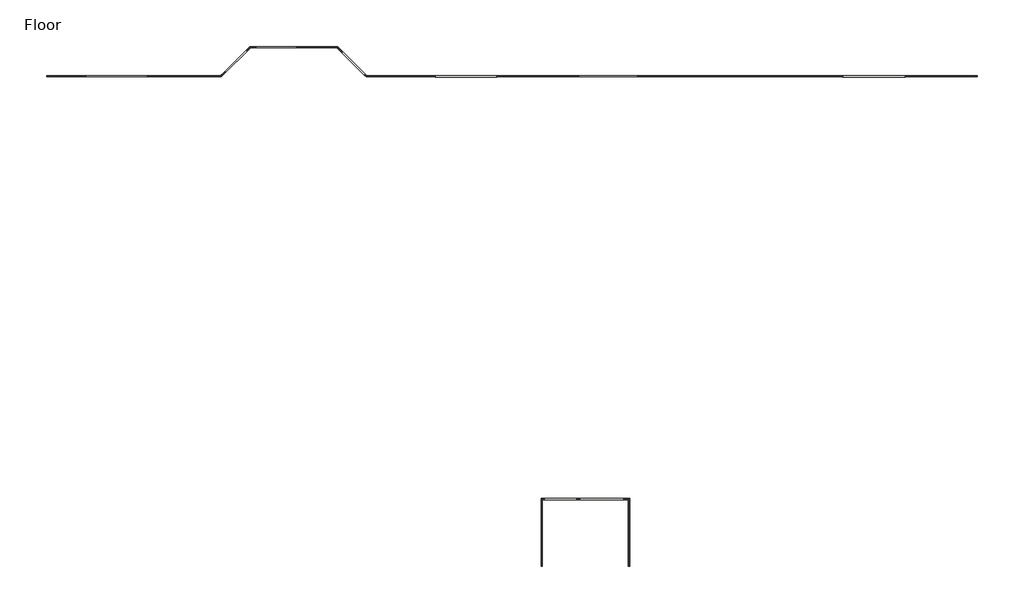
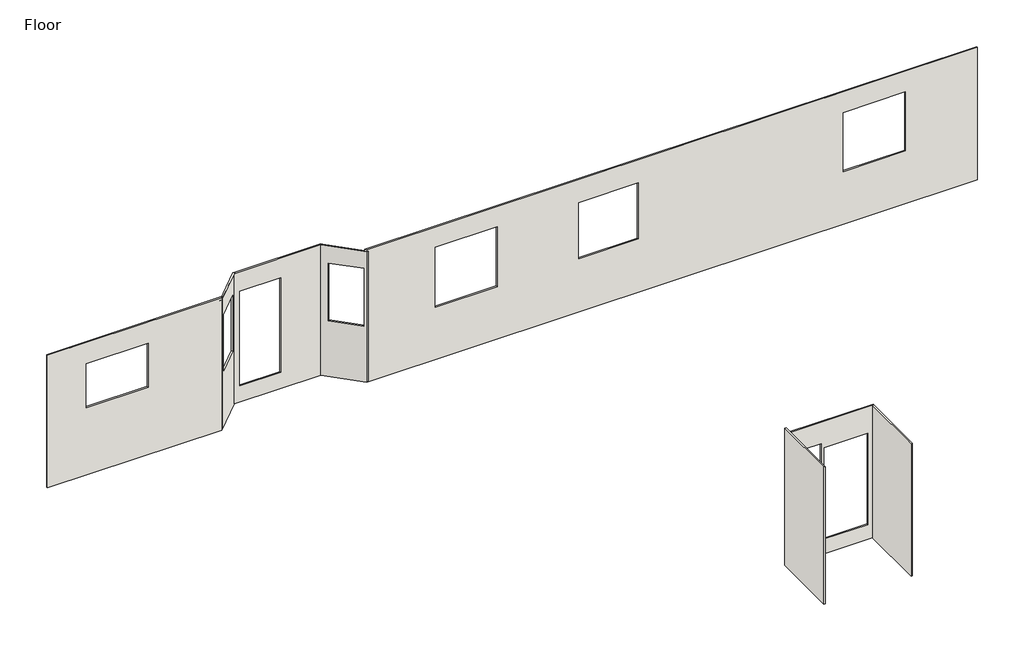
# One storey: 8 walls.
"""IFC4 building model written with IfcOpenShell, lengths in millimetres."""

import ifcopenshell
import ifcopenshell.guid

model = None  # the IFC model being written
_history = None  # IfcOwnerHistory: only IFC2X3 demands one
_inside = {}  # id of a spatial element -> (the spatial element, [elements in it])
_under = {}  # id of a project, library or spatial element -> (it, [spatial elements below it])
_declared = {}  # id of a project -> (the project, [libraries it declares])
_typed = {}  # id of a type object -> (the type object, [elements of that type])
_made_of = {}  # id of a material, layer set ... -> (it, [elements and type objects made of it])


def new_model(schema):
    """Start an empty IFC model of exactly this schema.

    Asked for "IFC4X3", IfcOpenShell would pick the latest addendum, in which some entities
    have other attributes; the version numbers below select the first issue.
    IFC2X3 requires an IfcOwnerHistory on every rooted entity: one is made here for all.
    """
    global model, _history
    if schema == "IFC4X3":
        model = ifcopenshell.file(schema_version=(4, 3, 0, 0))
    else:
        model = ifcopenshell.file(schema=schema)
    _inside.clear()
    _under.clear()
    _declared.clear()
    _typed.clear()
    _made_of.clear()
    _history = None
    if model.schema == "IFC2X3":
        org = make("IfcOrganization", Name="unknown")
        user = make(
            "IfcPersonAndOrganization",
            ThePerson=make("IfcPerson", FamilyName="unknown"),
            TheOrganization=org,
        )
        app = make(
            "IfcApplication",
            ApplicationDeveloper=org,
            Version="unknown",
            ApplicationFullName="unknown",
            ApplicationIdentifier="unknown",
        )
        _history = make(
            "IfcOwnerHistory",
            OwningUser=user,
            OwningApplication=app,
            ChangeAction="ADDED",
            CreationDate=0,
        )
    return model


def make(cls, **values):
    """One entity of the class cls with the attributes given. An attribute that is None is left unset."""
    return model.create_entity(
        cls, **{name: value for name, value in values.items() if value is not None}
    )


def rooted(cls, **values):
    """An entity with a GlobalId (a new one), such as an element, a storey or a relation."""
    return make(cls, GlobalId=ifcopenshell.guid.new(), OwnerHistory=_history, **values)


def si_unit(unit_type, name, prefix=None):
    """IfcSIUnit, for example si_unit("LENGTHUNIT", "METRE", prefix="MILLI")."""
    return make("IfcSIUnit", UnitType=unit_type, Prefix=prefix, Name=name)


def assignment(units):
    """IfcUnitAssignment: the units of a project."""
    return None if units is None else make("IfcUnitAssignment", Units=units)


def point(xyz):
    """IfcCartesianPoint."""
    return None if xyz is None else make("IfcCartesianPoint", Coordinates=xyz)


def direction(xyz):
    """IfcDirection."""
    return None if xyz is None else make("IfcDirection", DirectionRatios=xyz)


def frame(location, z_axis=None, x_axis=None):
    """IfcAxis2Placement3D, a coordinate frame: its origin and axes. An axis left out is left unset."""
    return make(
        "IfcAxis2Placement3D",
        Location=point(location),
        Axis=direction(z_axis),
        RefDirection=direction(x_axis),
    )


def origin():
    """The frame at (0, 0, 0) with its axes left unset."""
    return frame((0.0, 0.0, 0.0))


def place(relative_to, where):
    """IfcLocalPlacement: puts the frame where relative to a parent placement (None: the world)."""
    return make(
        "IfcLocalPlacement", PlacementRelTo=relative_to, RelativePlacement=where
    )


def context(
    kind, dimensions, precision=None, world=None, true_north=None, identifier=None
):
    """IfcGeometricRepresentationContext, for example the 3D "Model" context."""
    return make(
        "IfcGeometricRepresentationContext",
        ContextIdentifier=identifier,
        ContextType=kind,
        CoordinateSpaceDimension=dimensions,
        Precision=precision,
        WorldCoordinateSystem=world,
        TrueNorth=true_north,
    )


def project(units=None, contexts=None):
    """IfcProject with its units and contexts."""
    return rooted(
        "IfcProject",
        Name="project",
        RepresentationContexts=contexts,
        UnitsInContext=assignment(units),
    )


def spatial(cls, under=None, at=None, **own):
    """A site, building, storey or space (cls), placed at a placement, below another one or the project."""
    s = rooted(cls, ObjectPlacement=at, **own)
    if under is not None:
        _under.setdefault(under.id(), (under, []))[1].append(s)
    return s


def faces_of(points, faces, orient=None, outer=None):
    """IfcFace entities. A face is a list of loops; a loop is a list of indices into points, from 0.

    orient and outer hold one flag for each loop. By default every Orientation is true, the
    first loop of a face is its IfcFaceOuterBound and the others are IfcFaceBound.
    """
    made = []
    for i, loops in enumerate(faces):
        bounds = []
        for j, loop in enumerate(loops):
            is_outer = j == 0 if outer is None else outer[i][j]
            bounds.append(
                make(
                    "IfcFaceOuterBound" if is_outer else "IfcFaceBound",
                    Bound=make("IfcPolyLoop", Polygon=[points[k] for k in loop]),
                    Orientation=True if orient is None else orient[i][j],
                )
            )
        made.append(make("IfcFace", Bounds=bounds))
    return made


def faceted_brep(points, faces, orient=None, outer=None, voids=None):
    """IfcFacetedBrep: a solid bounded by flat faces; with voids (closed shells), ...WithVoids."""
    shared = [point(p) for p in points]
    hull = make("IfcClosedShell", CfsFaces=faces_of(shared, faces, orient, outer))
    if voids is None:
        return make("IfcFacetedBrep", Outer=hull)
    return make(
        "IfcFacetedBrepWithVoids",
        Outer=hull,
        Voids=[
            make(cls, CfsFaces=faces_of(shared, fs, o, b)) for cls, fs, o, b in voids
        ],
    )


def shape(context_of_items, identifier, shape_type, items):
    """IfcShapeRepresentation: the items that make up one representation, for example the "Body"."""
    return make(
        "IfcShapeRepresentation",
        ContextOfItems=context_of_items,
        RepresentationIdentifier=identifier,
        RepresentationType=shape_type,
        Items=items,
    )


def made_of(thing, what):
    """Note that an element or type object is made of a material, layer set ...; save() writes the relation."""
    if what is not None:
        _made_of.setdefault(what.id(), (what, []))[1].append(thing)
    return thing


def element(
    cls,
    number,
    at=None,
    inside=None,
    cuts=None,
    type_object=None,
    material=None,
    context=None,
    identifier="Body",
    shape_type=None,
    held_by="IfcProductDefinitionShape",
    body=None,
    shapes=None,
    **own,
):
    """One element of the class cls, such as IfcWall. Its Tag is "e" and its number.

    at: its placement. inside: the storey or other place that contains it. cuts: it is an
    opening in that element (IfcRelVoidsElement). A single representation is given by context,
    identifier, shape_type and body (its items); several are given by shapes. held_by: the class
    of the entity that holds the representations. save() writes the other relations.
    """
    e = rooted(cls, Tag="e%d" % number, ObjectPlacement=at, **own)
    if body is not None:
        shapes = [shape(context, identifier, shape_type, body)]
    if shapes is not None:
        e.Representation = make(held_by, Representations=shapes)
    if inside is not None:
        _inside.setdefault(inside.id(), (inside, []))[1].append(e)
    if cuts is not None:
        rooted(
            "IfcRelVoidsElement", RelatingBuildingElement=cuts, RelatedOpeningElement=e
        )
    if type_object is not None:
        _typed.setdefault(type_object.id(), (type_object, []))[1].append(e)
    return made_of(e, material)


def aggregate(whole, parts):
    """IfcRelAggregates: a whole, such as a stair, and the parts it consists of."""
    return rooted("IfcRelAggregates", RelatingObject=whole, RelatedObjects=parts)


def save(model, path):
    """Write the relations noted so far, then the file.

    IfcRelAggregates (storeys below a building ...), IfcRelContainedInSpatialStructure (elements
    in a storey), IfcRelDefinesByType, IfcRelAssociatesMaterial and IfcRelDeclares: one each for
    every whole, place, type object, material and project.
    """
    for whole, parts in _under.values():
        aggregate(whole, parts)
    for where, things in _inside.values():
        rooted(
            "IfcRelContainedInSpatialStructure",
            RelatedElements=things,
            RelatingStructure=where,
        )
    for kind, things in _typed.values():
        rooted("IfcRelDefinesByType", RelatedObjects=things, RelatingType=kind)
    for what, things in _made_of.values():
        rooted("IfcRelAssociatesMaterial", RelatedObjects=things, RelatingMaterial=what)
    for by, libraries in _declared.values():
        rooted("IfcRelDeclares", RelatingContext=by, RelatedDefinitions=libraries)
    model.write(path)


model = new_model("IFC4")

# Units and contexts
model_context = context("Model", 3, world=origin())
ifc_project = project(units=[si_unit("LENGTHUNIT", "METRE", prefix="MILLI")], contexts=[model_context])

# Site, building, storey
site = spatial("IfcSite", under=ifc_project)
building = spatial("IfcBuilding", under=site)
storey = spatial("IfcBuildingStorey", under=building, Name="Floor", Elevation=0.0)

# Walls
placement = place(None, origin())
element("IfcWall", 1, ObjectType="SIDING FINISHING", at=placement, inside=storey, context=model_context, shape_type="Brep", body=[
    faceted_brep([(-2566.5347564, 4527.226374, -339.725), (-6252.0152251, 4527.226374, -339.725), (-6252.0152251, 4527.226374, 2598.7952567), (-2566.5347564, 4527.226374, 2598.7952567), (-4140.2279723, 4527.226374, 2127.1715762), (-5435.5369686, 4527.226374, 2127.1715762), (-5435.5369686, 4527.226374, 1151.995982), (-4140.2279723, 4527.226374, 1151.995982), (-6252.0152251, 4499.3459053, -339.725), (-2594.4152251, 4499.3459053, -339.725), (-2594.4152251, 4499.3459053, 25.4), (-2594.4152251, 4499.3459053, 2598.7952567), (-6252.0152251, 4499.3459053, 2598.7952567), (-5435.5369686, 4499.3459053, 2127.1715762), (-4140.2279723, 4499.3459053, 2127.1715762), (-4140.2279723, 4499.3459053, 1151.995982), (-5435.5369686, 4499.3459053, 1151.995982)], [[[0, 1, 2, 3], [4, 5, 6, 7]], [[8, 9, 10, 11, 12], [13, 14, 15, 16]], [[1, 0, 9, 8]], [[3, 2, 12, 11]], [[2, 1, 8, 12]], [[0, 3, 11, 10, 9]], [[4, 14, 13, 5]], [[6, 16, 15, 7]], [[14, 4, 7, 15]], [[5, 13, 16, 6]]]),
])
element("IfcWall", 2, ObjectType="SIDING FINISHING", at=placement, inside=storey, context=model_context, shape_type="Brep", body=[
    faceted_brep([(13255.1847749, 4527.226374, -339.725), (416.6482831, 4527.226374, -339.725), (416.6482831, 4527.226374, 2598.7952567), (13255.1847749, 4527.226374, 2598.7952567), (13255.1847749, 4527.226374, -309.539672), (6140.6182584, 4527.226374, 2082.8), (4896.0182584, 4527.226374, 2082.8), (4896.0182584, 4527.226374, 839.7639243), (6140.6182584, 4527.226374, 839.7639243), (3184.311375, 4527.226374, 2144.4969986), (1888.4538423, 4527.226374, 2144.4969986), (1888.4538423, 4527.226374, 818.677442), (3184.311375, 4527.226374, 818.677442), (11745.8499153, 4527.226374, 2139.9865515), (10436.6397416, 4527.226374, 2139.9865515), (10436.6397416, 4527.226374, 830.7763778), (11745.8499153, 4527.226374, 830.7763778), (444.5287518, 4499.3459053, -339.725), (13255.1847749, 4499.3459053, -339.725), (13255.1847749, 4499.3459053, 2598.7952567), (444.5287518, 4499.3459053, 2598.7952567), (444.5287518, 4499.3459053, 0.0), (4896.0182584, 4499.3459053, 2082.8), (6140.6182584, 4499.3459053, 2082.8), (6140.6182584, 4499.3459053, 839.7639243), (4896.0182584, 4499.3459053, 839.7639243), (1888.4538423, 4499.3459053, 2144.4969986), (3184.311375, 4499.3459053, 2144.4969986), (3184.311375, 4499.3459053, 818.677442), (1888.4538423, 4499.3459053, 818.677442), (10436.6397416, 4499.3459053, 2139.9865515), (11745.8499153, 4499.3459053, 2139.9865515), (11745.8499153, 4499.3459053, 830.7763778), (10436.6397416, 4499.3459053, 830.7763778)], [[[0, 1, 2, 3, 4], [5, 6, 7, 8], [9, 10, 11, 12], [13, 14, 15, 16]], [[17, 18, 19, 20, 21], [22, 23, 24, 25], [26, 27, 28, 29], [30, 31, 32, 33]], [[1, 0, 18, 17]], [[3, 2, 20, 19]], [[0, 4, 3, 19, 18]], [[5, 23, 22, 6]], [[7, 25, 24, 8]], [[23, 5, 8, 24]], [[6, 22, 25, 7]], [[9, 27, 26, 10]], [[11, 29, 28, 12]], [[27, 9, 12, 28]], [[10, 26, 29, 11]], [[13, 31, 30, 14]], [[15, 33, 32, 16]], [[31, 13, 16, 32]], [[14, 30, 33, 15]], [[2, 1, 17, 21, 20]]]),
])
element("IfcWall", 3, ObjectType="SIDING FINISHING", at=placement, inside=storey, context=model_context, shape_type="Brep", body=[
    faceted_brep([(-1995.7323299, 5137.4577375, -339.725), (-2633.8441621, 4499.3459053, -339.725), (-2633.8441621, 4499.3459053, 2547.281212), (-1995.7323299, 5137.4577375, 2547.281212), (-2069.9596512, 5063.2304162, 2128.4354499), (-2518.9724573, 4614.2176101, 2128.4354499), (-2518.9724573, 4614.2176101, 889.0), (-2069.9596512, 5063.2304162, 889.0), (-2594.4152251, 4499.3459053, -339.725), (-1984.1838617, 5109.5772688, -339.725), (-1956.3033929, 5137.4577375, -339.725), (-1956.3033929, 5137.4577375, 2547.281212), (-1984.1838617, 5109.5772688, 2547.281212), (-2594.4152251, 4499.3459053, 2547.281212), (-2499.2579888, 4594.5031416, 2128.4354499), (-2050.2451827, 5043.5159477, 2128.4354499), (-2050.2451827, 5043.5159477, 889.0), (-2499.2579888, 4594.5031416, 889.0)], [[[0, 1, 2, 3], [4, 5, 6, 7]], [[8, 9, 10, 11, 12, 13], [14, 15, 16, 17]], [[1, 0, 10, 9, 8]], [[3, 2, 13, 12, 11]], [[2, 1, 8, 13]], [[4, 15, 14, 5]], [[6, 17, 16, 7]], [[15, 4, 7, 16]], [[5, 14, 17, 6]], [[0, 3, 11, 10]]]),
])
element("IfcWall", 4, ObjectType="SIDING FINISHING", at=placement, inside=storey, context=model_context, shape_type="Brep", body=[
    faceted_brep([(4139.0652436, -5762.2540947, -325.7586772), (4139.0652436, -4339.8540947, -325.7586772), (4139.0652436, -4339.8540947, 2598.7952567), (4139.0652436, -4339.8540947, 2717.8630484), (4139.0652436, -5762.2540947, 2717.8630484), (4139.0652436, -5762.2540947, 2649.5322083), (4111.1847749, -5762.2540947, -325.7586772), (4111.1847749, -5762.2540947, 2717.8630484), (4111.1847749, -4339.8540947, 2717.8630484), (4111.1847749, -4339.8540947, -325.7586772)], [[[0, 1, 2, 3, 4, 5]], [[6, 7, 8, 9]], [[1, 0, 6, 9]], [[4, 3, 8, 7]], [[0, 5, 4, 7, 6]], [[3, 2, 1, 9, 8]]]),
])
element("IfcWall", 5, ObjectType="SIDING FINISHING", at=placement, inside=storey, context=model_context, shape_type="Brep", body=[
    faceted_brep([(4139.0652436, -4367.7345635, -339.725), (5965.3847749, -4367.7345635, -339.725), (5965.3847749, -4367.7345635, 2598.7952567), (4139.0652436, -4367.7345635, 2598.7952567), (4926.4652436, -4367.7345635, 2014.5952567), (5838.3847749, -4367.7345635, 2014.5952567), (5838.3847749, -4367.7345635, -9.525), (4926.4652436, -4367.7345635, -9.525), (4174.1107589, -4367.7345635, 2127.1013961), (4857.2021617, -4367.7345635, 2127.1013961), (4857.2021617, -4367.7345635, 851.7342105), (4174.1107589, -4367.7345635, 851.7342105), (5965.3847749, -4339.8540947, -339.725), (4139.0652436, -4339.8540947, -339.725), (4139.0652436, -4339.8540947, -325.7586772), (4139.0652436, -4339.8540947, 2598.7952567), (5965.3847749, -4339.8540947, 2598.7952567), (5838.3847749, -4339.8540947, 2014.5952567), (4926.4652436, -4339.8540947, 2014.5952567), (4926.4652436, -4339.8540947, -9.525), (5838.3847749, -4339.8540947, -9.525), (4857.2021617, -4339.8540947, 2127.1013961), (4174.1107589, -4339.8540947, 2127.1013961), (4174.1107589, -4339.8540947, 851.7342105), (4857.2021617, -4339.8540947, 851.7342105)], [[[0, 1, 2, 3], [4, 5, 6, 7], [8, 9, 10, 11]], [[12, 13, 14, 15, 16], [17, 18, 19, 20], [21, 22, 23, 24]], [[1, 0, 13, 12]], [[3, 2, 16, 15]], [[2, 1, 12, 16]], [[0, 3, 15, 14, 13]], [[4, 18, 17, 5]], [[6, 20, 19, 7]], [[18, 4, 7, 19]], [[5, 17, 20, 6]], [[8, 22, 21, 9]], [[10, 24, 23, 11]], [[22, 8, 11, 23]], [[9, 21, 24, 10]]]),
])
element("IfcWall", 6, ObjectType="SIDING FINISHING", at=placement, inside=storey, context=model_context, shape_type="Brep", body=[
    faceted_brep([(5937.5043061, -4339.8540947, -339.725), (5937.5043061, -5762.2540947, -339.725), (5937.5043061, -5762.2540947, 2598.7952567), (5937.5043061, -4339.8540947, 2598.7952567), (5965.3847749, -4339.8540947, -339.725), (5965.3847749, -4339.8540947, 0.0), (5965.3847749, -4339.8540947, 2598.7952567), (5965.3847749, -5762.2540947, 2598.7952567), (5965.3847749, -5762.2540947, -339.725)], [[[0, 1, 2, 3]], [[4, 5, 6, 7, 8]], [[1, 0, 4, 8]], [[3, 2, 7, 6]], [[2, 1, 8, 7]], [[0, 3, 6, 5, 4]]]),
])
element("IfcWall", 7, ObjectType="SIDING FINISHING", at=placement, inside=storey, context=model_context, shape_type="Brep", body=[
    faceted_brep([(-154.1541434, 5137.4577375, -339.725), (-1956.3033929, 5137.4577375, -339.725), (-1956.3033929, 5137.4577375, 2547.281212), (-154.1541434, 5137.4577375, 2547.281212), (-1004.8982327, 5137.4577375, 2113.651697), (-1868.4982327, 5137.4577375, 2113.651697), (-1868.4982327, 5137.4577375, 15.875), (-1004.8982327, 5137.4577375, 15.875), (-1984.1838617, 5109.5772688, -339.725), (-165.7026117, 5109.5772688, -339.725), (-126.2736746, 5109.5772688, -339.725), (-126.2736746, 5109.5772688, 2547.281212), (-165.7026117, 5109.5772688, 2547.281212), (-1984.1838617, 5109.5772688, 2547.281212), (-1868.4982327, 5109.5772688, 2113.651697), (-1004.8982327, 5109.5772688, 2113.651697), (-1004.8982327, 5109.5772688, 15.875), (-1868.4982327, 5109.5772688, 15.875)], [[[0, 1, 2, 3], [4, 5, 6, 7]], [[8, 9, 10, 11, 12, 13], [14, 15, 16, 17]], [[1, 0, 10, 9, 8]], [[3, 2, 13, 12, 11]], [[2, 1, 8, 13]], [[0, 3, 11, 10]], [[4, 15, 14, 5]], [[6, 17, 16, 7]], [[15, 4, 7, 16]], [[5, 14, 17, 6]]]),
])
element("IfcWall", 8, ObjectType="SIDING FINISHING", at=placement, inside=storey, context=model_context, shape_type="Brep", body=[
    faceted_brep([(483.9576888, 4499.3459053, -339.725), (-126.2736746, 5109.5772688, -339.725), (-126.2736746, 5109.5772688, 2547.281212), (483.9576888, 4499.3459053, 2547.281212), (427.3857202, 4555.9178739, 2171.1003137), (-44.0777262, 5027.3813203, 2171.1003137), (-44.0777262, 5027.3813203, 889.0), (427.3857202, 4555.9178739, 889.0), (-165.7026117, 5109.5772688, -339.725), (444.5287518, 4499.3459053, -339.725), (444.5287518, 4499.3459053, 2547.281212), (-165.7026117, 5109.5772688, 2547.281212), (-63.7921947, 5007.6668518, 2171.1003137), (407.6712517, 4536.2034054, 2171.1003137), (407.6712517, 4536.2034054, 889.0), (-63.7921947, 5007.6668518, 889.0)], [[[0, 1, 2, 3], [4, 5, 6, 7]], [[8, 9, 10, 11], [12, 13, 14, 15]], [[1, 0, 9, 8]], [[3, 2, 11, 10]], [[2, 1, 8, 11]], [[0, 3, 10, 9]], [[4, 13, 12, 5]], [[6, 15, 14, 7]], [[13, 4, 7, 14]], [[5, 12, 15, 6]]]),
])

save(model, "model.ifc")

# Revit data of these elements
# Project information
#   Project Issue Date = "2022-10-14"
#   Project Status = "Project Status"
#   Client Name = "Owner"
#   Project Address = "Enter address here"
#   Project Name = "JOHNSON RESIDENCE"
#   Project Number = "01"
# Grids (mm)
#   "B": line (16433.72, 517.896) -> (-9340.445, 517.896)
#   "2": line (412.31, 6818.592) -> (412.31, -8454.654)
#   "3": line (4055.622, 6818.592) -> (4055.622, -8454.654)
#   "4": line (6052.697, 6818.592) -> (6052.697, -8454.654)
#   "5": line (9597.585, 6818.592) -> (9597.585, -8454.654)
#   "6": line (13255.185, 6818.592) -> (13255.185, -8454.654)
#   "1": line (-6252.015, 6818.592) -> (-6252.015, -6811.379)
#   "A": line (-9340.445, 4499.346) -> (14913.888, 4499.346)
#   "D": line (-9284.088, -5705.898) -> (14970.244, -5705.898)
#   "C": line (-9340.445, -1545.854) -> (17369.985, -1545.854)
# Type "SIDING FINISHING"
#   Keynote = "F10"
#   Layers, outside or top first: 0' - 1 9/256" "Aluminum double-6 siding" (function 4); 0' - 0 1/16" "Aluminum double-6 siding" (function 1)
# Elements 1, 2, 5, 6 (IfcWall, "SIDING FINISHING")
#   built-in parameter 1001111 = -1' - 1 3/8"
#   Top Offset = -0' - 1.99752"
#   Base Offset = -1' - 1 3/8"
#   wall height = 9' - 7.68977"
#   Phase Created = New Construction
#   Base Constraint = Floor
#   Top Constraint = Siding Wall
#   Materials on its faces: "Aluminum double-6 siding"
# Elements 3, 7, 8 (IfcWall, "SIDING FINISHING")
#   built-in parameter 1001111 = -1' - 1 3/8"
#   Top Offset = -0' - 4.02563"
#   Base Offset = -1' - 1 3/8"
#   wall height = 9' - 5.66166"
#   Phase Created = New Construction
#   Base Constraint = Floor
#   Top Constraint = Siding Wall
#   Materials on its faces: "Aluminum double-6 siding"
# Element 4 (IfcWall, "SIDING FINISHING")
#   built-in parameter 1001111 = -1' - 0.82514"
#   Top Offset = 0' - 2.69019"
#   Base Offset = -1' - 0.82514"
#   wall height = 9' - 11.82763"
#   Phase Created = New Construction
#   Base Constraint = Floor
#   Top Constraint = Siding Wall
#   Materials on its faces: "Aluminum double-6 siding"
# Materials
#   "Aluminum double-6 siding": class "Wood", colour RGB 205 199 197, transparency 0, Description = "Softwood clapboard siding", Cost = 0
